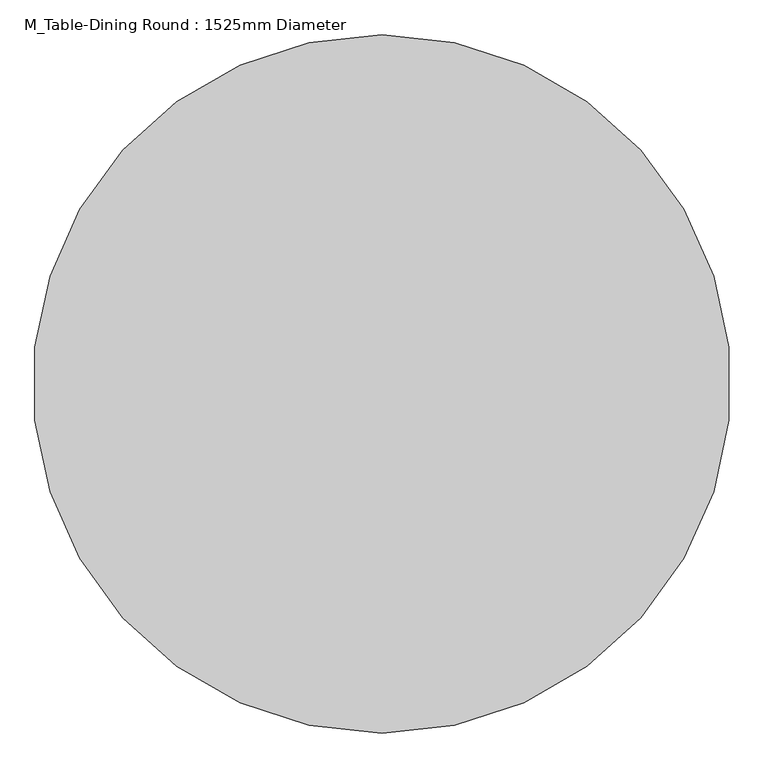
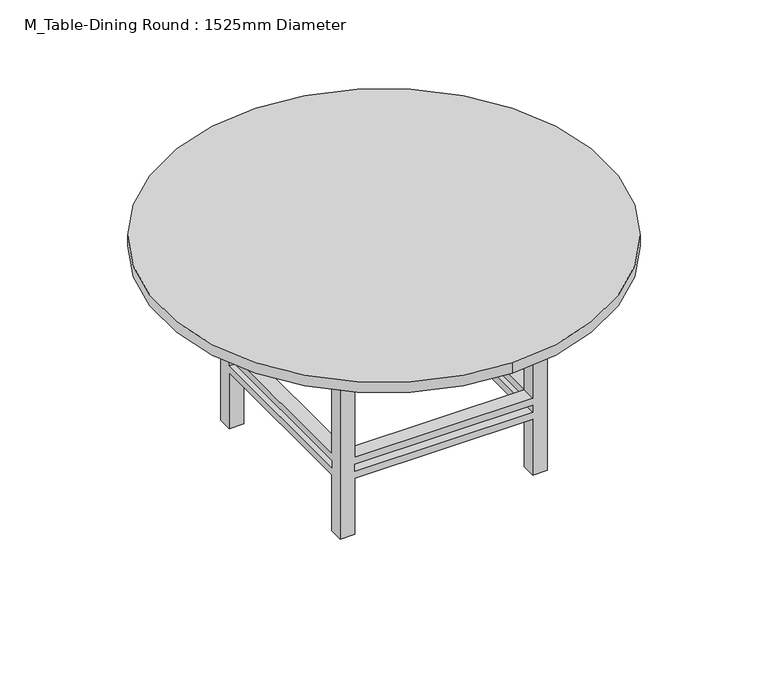
"""IFC4 building model written with IfcOpenShell, lengths in millimetres: furniture geometry, M_Table-Dining Round : 1525mm Diameter."""

from ifc_helpers import new_model, si_unit, point, frame, frame_2d, origin, place, context, project, spatial, polyline, circle_curve, trimmed, segment, composite_curve, outline, extrude, faceted_brep, source, transform, mapped, element, save


def m_table_dining_round_1525mm_diameter_e8096f67(model_context):
    return source(origin(), model_context, "Body", "SolidModel", [
        faceted_brep([(-201.3680328, 170.9713115, 647.7), (-252.1680328, 170.9713115, 647.7), (-252.1680328, 120.1713115, 647.7), (-201.3680328, 120.1713115, 647.7), (408.7319672, 170.9713115, 647.7), (408.7319672, 120.1713115, 647.7), (459.5319672, 120.1713115, 647.7), (459.5319672, 170.9713115, 647.7), (408.7319672, -540.7286885, 647.7), (459.5319672, -540.7286885, 647.7), (459.5319672, -489.9286885, 647.7), (408.7319672, -489.9286885, 647.7), (-201.3680328, -540.7286885, 647.7), (-201.3680328, -489.9286885, 647.7), (-252.1680328, -489.9286885, 647.7), (-252.1680328, -540.7286885, 647.7), (-201.3680328, 170.9713115, 0.0), (-201.3680328, 120.1713115, 0.0), (-252.1680328, 120.1713115, 0.0), (-252.1680328, 170.9713115, 0.0), (408.7319672, 170.9713115, 0.0), (459.5319672, 170.9713115, 0.0), (459.5319672, 120.1713115, 0.0), (408.7319672, 120.1713115, 0.0), (408.7319672, -540.7286885, 0.0), (408.7319672, -489.9286885, 0.0), (459.5319672, -489.9286885, 0.0), (459.5319672, -540.7286885, 0.0), (-201.3680328, -540.7286885, 0.0), (-252.1680328, -540.7286885, 0.0), (-252.1680328, -489.9286885, 0.0), (-201.3680328, -489.9286885, 0.0), (-201.3680328, 170.9713115, 279.4), (408.7319672, 170.9713115, 279.4), (408.7319672, 170.9713115, 203.2), (-201.3680328, 170.9713115, 203.2), (408.7319672, 170.9713115, 228.6), (408.7319672, 170.9713115, 254.0), (-201.3680328, 170.9713115, 254.0), (-201.3680328, 170.9713115, 228.6), (-252.1680328, 120.1713115, 203.2), (-252.1680328, -489.9286885, 203.2), (-252.1680328, -489.9286885, 279.4), (-252.1680328, 120.1713115, 279.4), (-252.1680328, 120.1713115, 228.6), (-252.1680328, 120.1713115, 254.0), (-252.1680328, -489.9286885, 254.0), (-252.1680328, -489.9286885, 228.6), (-201.3680328, 120.1713115, 279.4), (-201.3680328, 120.1713115, 203.2), (-201.3680328, 120.1713115, 228.6), (-201.3680328, 120.1713115, 254.0), (408.7319672, 120.1713115, 279.4), (408.7319672, 120.1713115, 203.2), (408.7319672, 120.1713115, 228.6), (408.7319672, 120.1713115, 254.0), (459.5319672, 120.1713115, 279.4), (459.5319672, 120.1713115, 203.2), (459.5319672, 120.1713115, 228.6), (459.5319672, 120.1713115, 254.0), (459.5319672, -489.9286885, 279.4), (459.5319672, -489.9286885, 203.2), (459.5319672, -489.9286885, 228.6), (459.5319672, -489.9286885, 254.0), (408.7319672, -540.7286885, 279.4), (-201.3680328, -540.7286885, 279.4), (-201.3680328, -540.7286885, 203.2), (408.7319672, -540.7286885, 203.2), (-201.3680328, -540.7286885, 228.6), (-201.3680328, -540.7286885, 254.0), (408.7319672, -540.7286885, 254.0), (408.7319672, -540.7286885, 228.6), (408.7319672, -489.9286885, 279.4), (408.7319672, -489.9286885, 203.2), (408.7319672, -489.9286885, 228.6), (408.7319672, -489.9286885, 254.0), (-201.3680328, -489.9286885, 279.4), (-201.3680328, -489.9286885, 203.2), (-201.3680328, -489.9286885, 228.6), (-201.3680328, -489.9286885, 254.0)], [[[0, 1, 2, 3]], [[4, 5, 6, 7]], [[8, 9, 10, 11]], [[12, 13, 14, 15]], [[16, 17, 18, 19]], [[20, 21, 22, 23]], [[24, 25, 26, 27]], [[28, 29, 30, 31]], [[1, 0, 32, 33, 4, 7, 21, 20, 34, 35, 16, 19], [36, 37, 38, 39]], [[2, 1, 19, 18, 40, 41, 30, 29, 15, 14, 42, 43], [44, 45, 46, 47]], [[3, 2, 43, 48]], [[18, 17, 49, 40]], [[44, 50, 51, 45]], [[0, 3, 48, 32]], [[17, 16, 35, 49]], [[50, 39, 38, 51]], [[5, 4, 33, 52]], [[20, 23, 53, 34]], [[36, 54, 55, 37]], [[6, 5, 52, 56]], [[23, 22, 57, 53]], [[54, 58, 59, 55]], [[21, 7, 6, 56, 60, 10, 9, 27, 26, 61, 57, 22], [62, 63, 59, 58]], [[27, 9, 8, 64, 65, 12, 15, 29, 28, 66, 67, 24], [68, 69, 70, 71]], [[11, 10, 60, 72]], [[26, 25, 73, 61]], [[62, 74, 75, 63]], [[8, 11, 72, 64]], [[25, 24, 67, 73]], [[74, 71, 70, 75]], [[13, 12, 65, 76]], [[28, 31, 77, 66]], [[68, 78, 79, 69]], [[14, 13, 76, 42]], [[31, 30, 41, 77]], [[78, 47, 46, 79]], [[54, 74, 62, 58]], [[74, 78, 68, 71]], [[78, 50, 44, 47]], [[50, 54, 36, 39]], [[53, 49, 35, 34]], [[49, 77, 41, 40]], [[77, 73, 67, 66]], [[73, 53, 57, 61]], [[74, 54, 53, 73]], [[78, 74, 73, 77]], [[50, 78, 77, 49]], [[54, 50, 49, 53]], [[52, 72, 60, 56]], [[72, 76, 65, 64]], [[76, 48, 43, 42]], [[48, 52, 33, 32]], [[55, 51, 38, 37]], [[51, 79, 46, 45]], [[79, 75, 70, 69]], [[75, 55, 59, 63]], [[72, 52, 55, 75]], [[76, 72, 75, 79]], [[48, 76, 79, 51]], [[52, 48, 51, 55]]]),
        extrude(outline(polyline([(484.9319672, 196.3713115), (484.9319672, -566.1286885), (-277.5680328, -566.1286885), (-277.5680328, 196.3713115), (484.9319672, 196.3713115)]), holes=[polyline([(459.5319672, 170.9713115), (-252.1680328, 170.9713115), (-252.1680328, -540.7286885), (459.5319672, -540.7286885), (459.5319672, 170.9713115)])]), frame((0.0, 0.0, 647.7), z_axis=(0.0, 0.0, 1.0), x_axis=(1.0, 0.0, 0.0)), (0.0, 0.0, 1.0), 76.2),
        extrude(outline(composite_curve([segment(trimmed(circle_curve(frame_2d((103.6819672, -184.8786885)), 762.5), [point((103.6819672, -947.3786885))], [point((103.6819672, 577.6213115))], False, "CARTESIAN"), True, "CONTINUOUS"), segment(trimmed(circle_curve(frame_2d((103.6819672, -184.8786885)), 762.5), [point((103.6819672, 577.6213115))], [point((103.6819672, -947.3786885))], False, "CARTESIAN"), True, "CONTINUOUS")], self_intersect=False)), frame((0.0, 0.0, 723.9), z_axis=(0.0, 0.0, 1.0), x_axis=(1.0, 0.0, 0.0)), (0.0, 0.0, 1.0), 38.1),
    ])


if __name__ == "__main__":
    model = new_model("IFC4")
    model_context = context("Model", 3, world=origin())
    ifc_project = project(units=[si_unit("LENGTHUNIT", "METRE", prefix="MILLI")], contexts=[model_context])
    site = spatial("IfcSite", under=ifc_project)
    building = spatial("IfcBuilding", under=site)
    placement = place(None, origin())
    m_table_dining_round_1525mm_diameter_shape = m_table_dining_round_1525mm_diameter_e8096f67(model_context)
    element("IfcFurniture", 1, ObjectType="M_Table-Dining Round : 1525mm Diameter", at=placement, inside=building, context=model_context, shape_type="MappedRepresentation", body=[
        mapped(m_table_dining_round_1525mm_diameter_shape, transform((0.0, 0.0, 0.0), x_axis=(1.0, 0.0, 0.0), y_axis=(0.0, 1.0, 0.0), z_axis=(0.0, 0.0, 1.0))),
    ])
    save(model, "model.ifc")

# Revit data of these elements
# Type "M_Table-Dining Round : 1525mm Diameter"
#   Diameter = 1.525 m
#   Height = 0.762 m
#   Base Material = Pine
#   Top Material = Laminate, Linen, Matte
# Element 1 (IfcFurniture, "M_Table-Dining Round : 1525mm Diameter")
#   Materials on its faces: "Pine", "Laminate, Linen, Matte"
# Materials
#   "Pine": class "Wood", colour RGB 223 192 134, transparency 0, Description = "Pinus Echinata", Cost = 0
#   "Laminate, Linen, Matte": class "Plastic", colour RGB 249 239 230, transparency 0, Description = "Laminado de plástico - Lino, mate", Cost = 0
